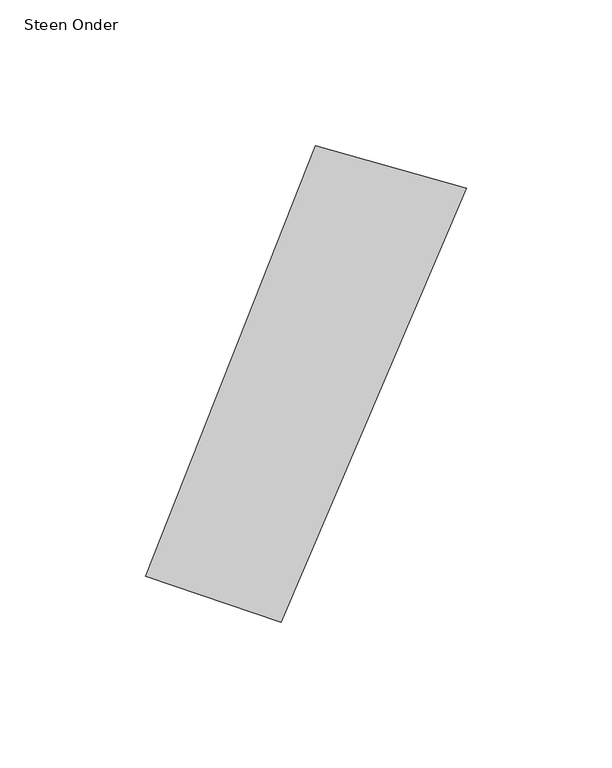
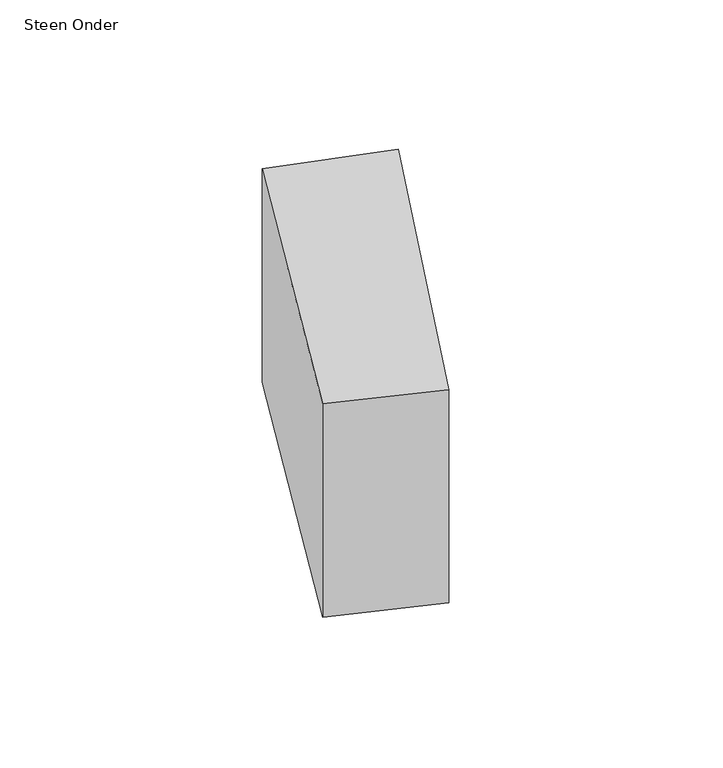
"""IFC4 building model written with IfcOpenShell, lengths in millimetres: proxy geometry, 00_GMA_steen_versie_4 : Steen Onder."""

from ifc_helpers import new_model, si_unit, origin, origin_with_axes, place, context, project, spatial, polyline, outline, extrude, source, transform, mapped, element, save


def steen_onder_23840e80(model_context):
    return source(origin(), model_context, "Body", "SweptSolid", [
        extrude(outline(polyline([(131.680733, 142.4948935), (68.0023028, -6.6891915), (21.3315402, 9.1770252), (79.8415926, 157.1394843), (131.680733, 142.4948935)])), origin_with_axes(), (0.0, 0.0, 1.0), 100.0),
    ])


if __name__ == "__main__":
    model = new_model("IFC4")
    model_context = context("Model", 3, world=origin())
    ifc_project = project(units=[si_unit("LENGTHUNIT", "METRE", prefix="MILLI")], contexts=[model_context])
    site = spatial("IfcSite", under=ifc_project)
    building = spatial("IfcBuilding", under=site)
    placement = place(None, origin())
    steen_onder_shape = steen_onder_23840e80(model_context)
    element("IfcBuildingElementProxy", 1, Name="00_GMA_steen_versie_4 : Steen Onder", ObjectType="00_GMA_steen_versie_4 : Steen Onder", at=placement, inside=building, context=model_context, shape_type="MappedRepresentation", body=[
        mapped(steen_onder_shape, transform((0.0, 0.0, 0.0), x_axis=(1.0, 0.0, 0.0), y_axis=(0.0, 1.0, 0.0), z_axis=(0.0, 0.0, 1.0))),
    ])
    save(model, "model.ifc")

# Revit data of these elements
# Type "00_GMA_steen_versie_4 : Steen Onder"
#   StootVoegHalfBoven [instance default] = 5 mm
#   StootVoegHalf [instance default] = 5 mm
#   StootVoegBreedteOnder = 10 mm
#   StootVoegBreedteBoven = 10 mm
#   Steendikte = 100 mm
#   LintVoegOnderHalf = 0 mm
#   LintVoegOnder = 0 mm
#   LintVoegBovenHalf = 5 mm
#   LintVoegBoven = 10 mm
#   materiaal = none
#   MateriaalVoeg = none
#   Default Elevation = 0
